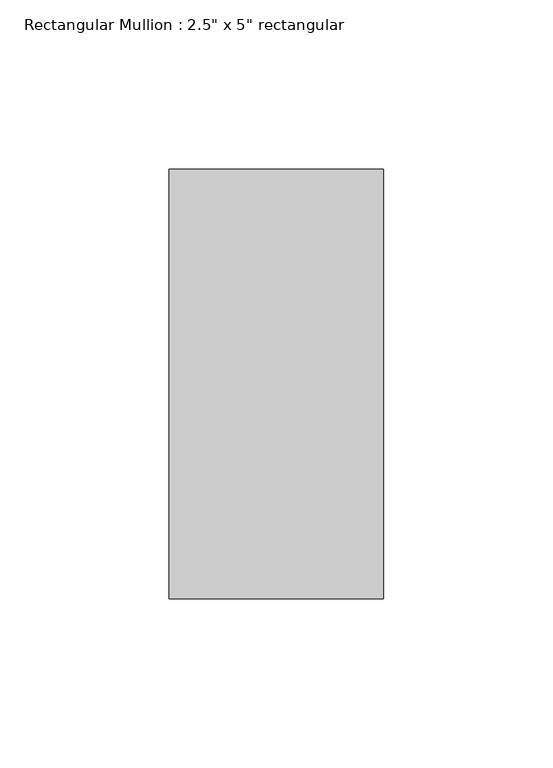
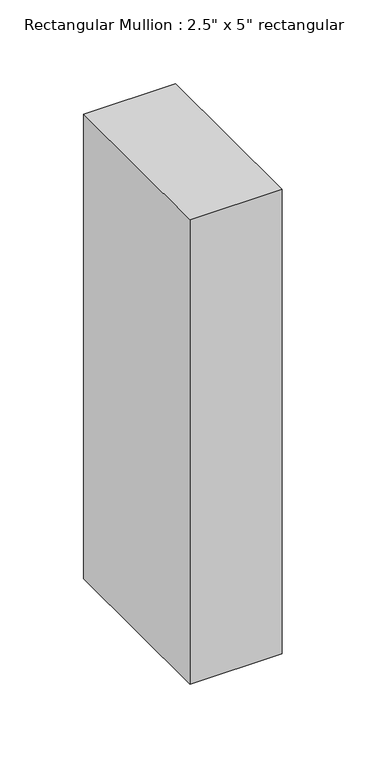
"""IFC4 building model written with IfcOpenShell, lengths in millimetres: member geometry."""

from ifc_helpers import new_model, si_unit, frame, origin, place, context, project, spatial, polyline, outline, extrude, source, transform, mapped, element, save


def member_a4308164(model_context):
    return source(origin(), model_context, "Body", "SweptSolid", [
        extrude(outline(polyline([(0.0, 63.5), (0.0, -63.5), (-63.5, -63.5), (-63.5, 63.5), (0.0, 63.5)])), frame((0.0, 0.0, -338.3578591), z_axis=(0.0, 0.0, 1.0), x_axis=(1.0, 0.0, 0.0)), (0.0, 0.0, 1.0), 338.3578591),
    ])


if __name__ == "__main__":
    model = new_model("IFC4")
    model_context = context("Model", 3, world=origin())
    ifc_project = project(units=[si_unit("LENGTHUNIT", "METRE", prefix="MILLI")], contexts=[model_context])
    site = spatial("IfcSite", under=ifc_project)
    building = spatial("IfcBuilding", under=site)
    placement = place(None, origin())
    member_shape = member_a4308164(model_context)
    element("IfcMember", 1, ObjectType="Rectangular Mullion : 2.5\" x 5\" rectangular", at=placement, inside=building, context=model_context, shape_type="MappedRepresentation", body=[
        mapped(member_shape, transform((0.0, 0.0, 0.0), x_axis=(1.0, 0.0, 0.0), y_axis=(0.0, 1.0, 0.0), z_axis=(0.0, 0.0, 1.0))),
    ])
    save(model, "model.ifc")

# Revit data of these elements
# Type "Rectangular Mullion : 2.5\" x 5\" rectangular"
#   built-in parameter 1007304 = 0.416667 (stored number, unit not read)
#   built-in parameter 1007301 = 0.104167 (stored number, unit not read)
#   built-in parameter 1007300 = 0.104167 (stored number, unit not read)
# Element 1 (IfcMember, "Rectangular Mullion : 2.5\" x 5\" rectangular")
#   Materials on its faces: "Metal - Aluminum 2"
# Materials
#   "Metal - Aluminum 2": class "Metal", colour RGB 189 187 185, transparency 0
